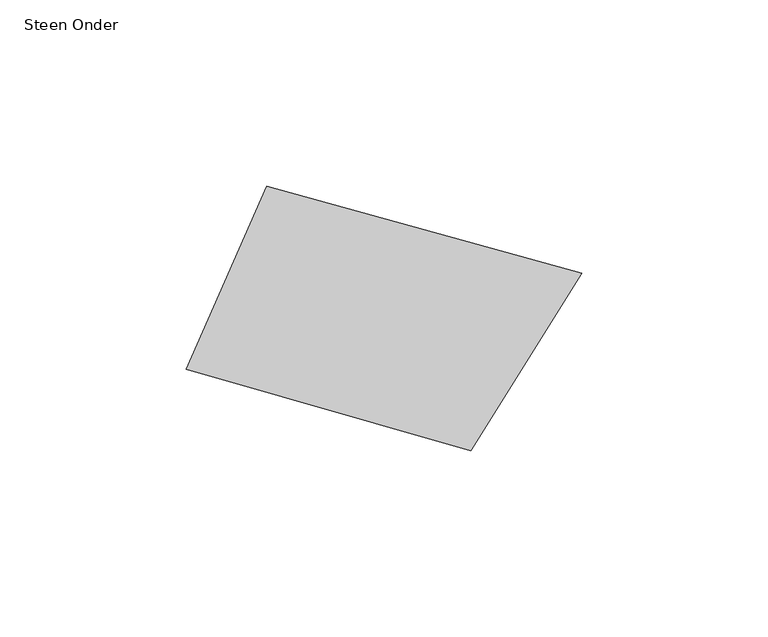
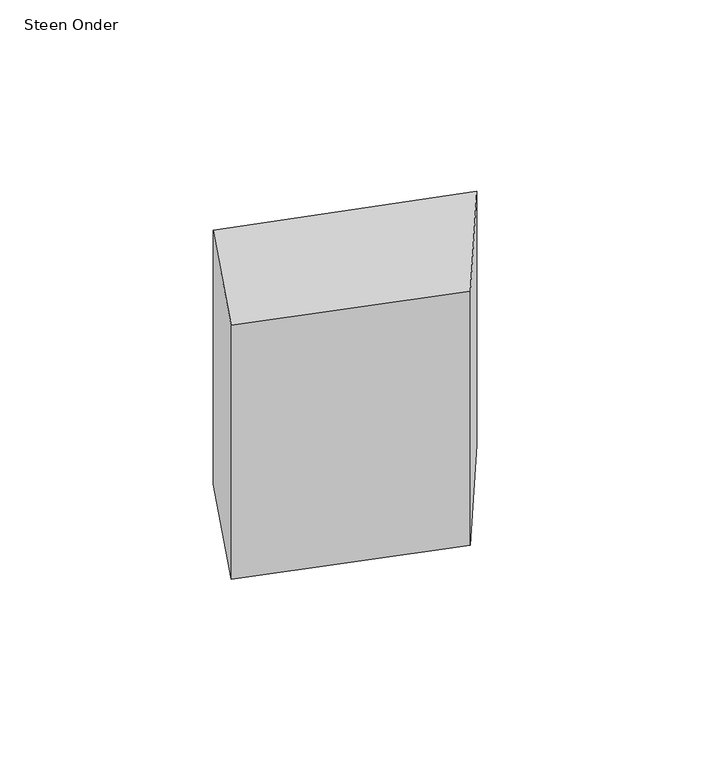
"""IFC4 building model written with IfcOpenShell, lengths in millimetres: proxy geometry, 00_GMA_steen_versie_4 : Steen Onder."""

from ifc_helpers import new_model, si_unit, frame, origin, place, context, project, spatial, polyline, outline, extrude, source, transform, mapped, element, save


def steen_onder_9ebafeed(model_context):
    return source(origin(), model_context, "Body", "SweptSolid", [
        extrude(outline(polyline([(143.308548, 53.0769471), (113.4129976, 5.4179246), (37.003099, 27.3169139), (58.6285004, 76.5086938), (143.308548, 53.0769471)])), frame((0.0, 0.0, -100.0), z_axis=(0.0, 0.0, 1.0), x_axis=(1.0, 0.0, 0.0)), (0.0, 0.0, 1.0), 100.0),
    ])


if __name__ == "__main__":
    model = new_model("IFC4")
    model_context = context("Model", 3, world=origin())
    ifc_project = project(units=[si_unit("LENGTHUNIT", "METRE", prefix="MILLI")], contexts=[model_context])
    site = spatial("IfcSite", under=ifc_project)
    building = spatial("IfcBuilding", under=site)
    placement = place(None, origin())
    steen_onder_shape = steen_onder_9ebafeed(model_context)
    element("IfcBuildingElementProxy", 1, Name="00_GMA_steen_versie_4 : Steen Onder", ObjectType="00_GMA_steen_versie_4 : Steen Onder", at=placement, inside=building, context=model_context, shape_type="MappedRepresentation", body=[
        mapped(steen_onder_shape, transform((0.0, 0.0, 0.0), x_axis=(1.0, 0.0, 0.0), y_axis=(0.0, 1.0, 0.0), z_axis=(0.0, 0.0, 1.0))),
    ])
    save(model, "model.ifc")

# Revit data of these elements
# Type "00_GMA_steen_versie_4 : Steen Onder"
#   StootVoegHalfBoven [instance default] = 5 mm
#   StootVoegHalf [instance default] = 5 mm
#   StootVoegBreedteOnder = 10 mm
#   StootVoegBreedteBoven = 10 mm
#   Steendikte = 100 mm
#   LintVoegOnderHalf = 0 mm
#   LintVoegOnder = 0 mm
#   LintVoegBovenHalf = 5 mm
#   LintVoegBoven = 10 mm
#   materiaal = none
#   MateriaalVoeg = none
#   Default Elevation = 0
